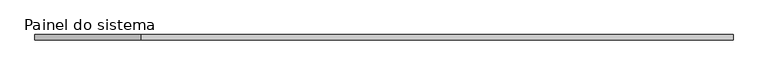
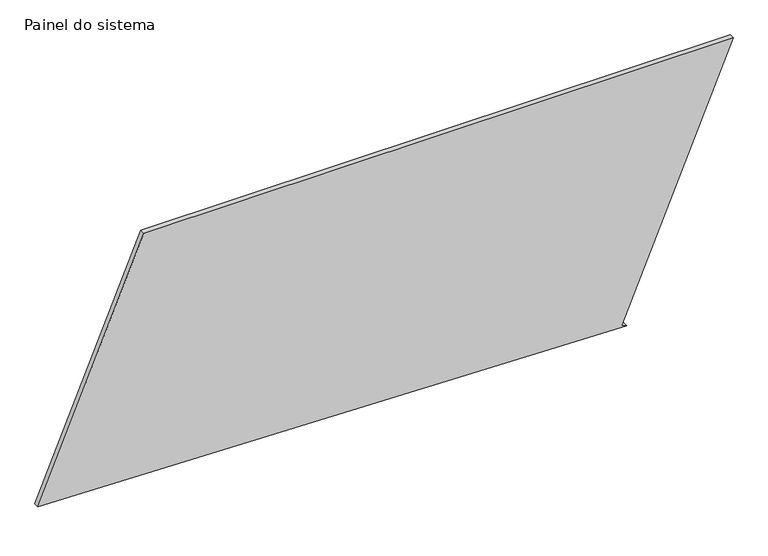
"""IFC4 building model written with IfcOpenShell, lengths in millimetres: plate geometry, Painel do sistema : Envidraçado."""

from ifc_helpers import new_model, si_unit, frame, origin, place, context, project, spatial, polyline, outline, extrude, source, transform, mapped, element, save


def painel_do_sistema_8e512fd9(model_context):
    return source(origin(), model_context, "Body", "SweptSolid", [
        extrude(outline(polyline([(0.0, 1131.4943233), (9.6723918, 1108.4412359), (1251.896626, 1629.6416843), (1251.896626, -1133.1433088), (68.5470795, -1629.6416843), (0.0, 1131.4943233)])), frame((0.0, 24.5, 0.0), z_axis=(0.0, 1.0, 0.0), x_axis=(0.0, 0.0, 1.0)), (0.0, 0.0, 1.0), 25.0),
    ])


if __name__ == "__main__":
    model = new_model("IFC4")
    model_context = context("Model", 3, world=origin())
    ifc_project = project(units=[si_unit("LENGTHUNIT", "METRE", prefix="MILLI")], contexts=[model_context])
    site = spatial("IfcSite", under=ifc_project)
    building = spatial("IfcBuilding", under=site)
    placement = place(None, origin())
    painel_do_sistema_shape = painel_do_sistema_8e512fd9(model_context)
    element("IfcPlate", 1, ObjectType="Painel do sistema : Envidraçado", at=placement, inside=building, context=model_context, shape_type="MappedRepresentation", body=[
        mapped(painel_do_sistema_shape, transform((0.0, 0.0, 0.0), x_axis=(1.0, 0.0, 0.0), y_axis=(0.0, 1.0, 0.0), z_axis=(0.0, 0.0, 1.0))),
    ])
    save(model, "model.ifc")

# Revit data of these elements
# Type "Painel do sistema : Envidraçado"
#   Construction Type Id = "GSP4R"
#   Analytic Construction = "Vidraça única Pilkington 1/8 pol"
#   Visual Light Transmittance = 0.9
#   Solar Heat Gain Coefficient = 0.86
#   Heat Transfer Coefficient (U) = 6.7069 W/(m²·K)
# Element 1 (IfcPlate, "Painel do sistema : Envidraçado")
#   Materials on its faces: "Vidro"
# Materials
#   "Vidro": class "Vidro", colour RGB 0 128 192, transparency 0.9, Description = "Vidro de sílica", Cost = 0
